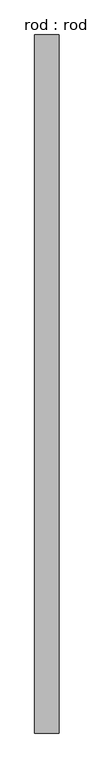
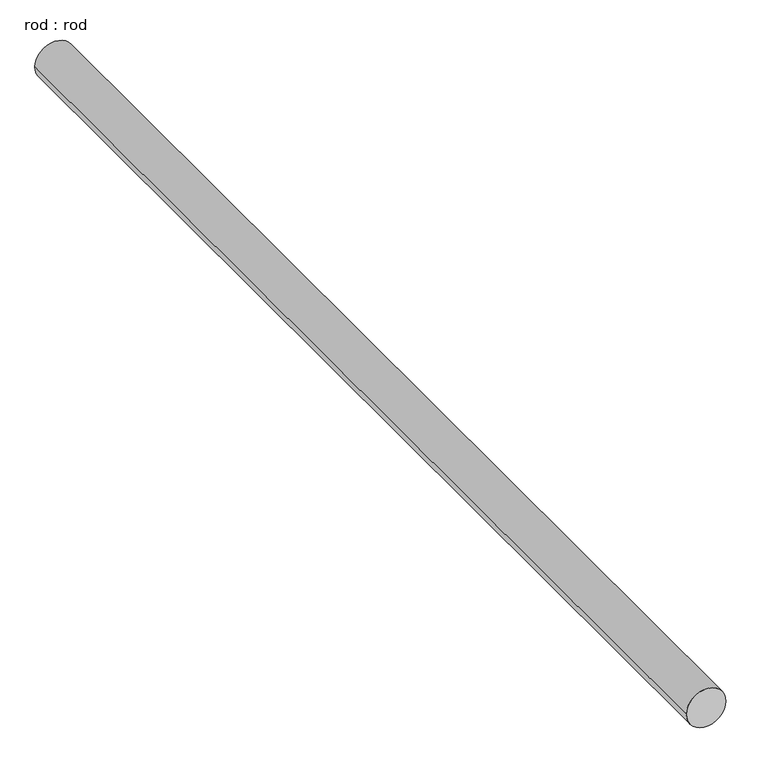
"""IFC4 building model written with IfcOpenShell, lengths in millimetres: proxy geometry, rod : rod."""

import ifcopenshell
import ifcopenshell.guid

model = None  # the IFC model being written
_history = None  # IfcOwnerHistory: only IFC2X3 demands one
_inside = {}  # id of a spatial element -> (the spatial element, [elements in it])
_under = {}  # id of a project, library or spatial element -> (it, [spatial elements below it])
_declared = {}  # id of a project -> (the project, [libraries it declares])
_typed = {}  # id of a type object -> (the type object, [elements of that type])
_made_of = {}  # id of a material, layer set ... -> (it, [elements and type objects made of it])


def new_model(schema):
    """Start an empty IFC model of exactly this schema.

    Asked for "IFC4X3", IfcOpenShell would pick the latest addendum, in which some entities
    have other attributes; the version numbers below select the first issue.
    IFC2X3 requires an IfcOwnerHistory on every rooted entity: one is made here for all.
    """
    global model, _history
    if schema == "IFC4X3":
        model = ifcopenshell.file(schema_version=(4, 3, 0, 0))
    else:
        model = ifcopenshell.file(schema=schema)
    _inside.clear()
    _under.clear()
    _declared.clear()
    _typed.clear()
    _made_of.clear()
    _history = None
    if model.schema == "IFC2X3":
        org = make("IfcOrganization", Name="unknown")
        user = make(
            "IfcPersonAndOrganization",
            ThePerson=make("IfcPerson", FamilyName="unknown"),
            TheOrganization=org,
        )
        app = make(
            "IfcApplication",
            ApplicationDeveloper=org,
            Version="unknown",
            ApplicationFullName="unknown",
            ApplicationIdentifier="unknown",
        )
        _history = make(
            "IfcOwnerHistory",
            OwningUser=user,
            OwningApplication=app,
            ChangeAction="ADDED",
            CreationDate=0,
        )
    return model


def make(cls, **values):
    """One entity of the class cls with the attributes given. An attribute that is None is left unset."""
    return model.create_entity(
        cls, **{name: value for name, value in values.items() if value is not None}
    )


def rooted(cls, **values):
    """An entity with a GlobalId (a new one), such as an element, a storey or a relation."""
    return make(cls, GlobalId=ifcopenshell.guid.new(), OwnerHistory=_history, **values)


def si_unit(unit_type, name, prefix=None):
    """IfcSIUnit, for example si_unit("LENGTHUNIT", "METRE", prefix="MILLI")."""
    return make("IfcSIUnit", UnitType=unit_type, Prefix=prefix, Name=name)


def assignment(units):
    """IfcUnitAssignment: the units of a project."""
    return None if units is None else make("IfcUnitAssignment", Units=units)


def point(xyz):
    """IfcCartesianPoint."""
    return None if xyz is None else make("IfcCartesianPoint", Coordinates=xyz)


def direction(xyz):
    """IfcDirection."""
    return None if xyz is None else make("IfcDirection", DirectionRatios=xyz)


def frame(location, z_axis=None, x_axis=None):
    """IfcAxis2Placement3D, a coordinate frame: its origin and axes. An axis left out is left unset."""
    return make(
        "IfcAxis2Placement3D",
        Location=point(location),
        Axis=direction(z_axis),
        RefDirection=direction(x_axis),
    )


def frame_2d(location, x_axis=None):
    """IfcAxis2Placement2D, a coordinate frame in the plane: its origin and x axis."""
    return make(
        "IfcAxis2Placement2D", Location=point(location), RefDirection=direction(x_axis)
    )


def origin():
    """The frame at (0, 0, 0) with its axes left unset."""
    return frame((0.0, 0.0, 0.0))


def place(relative_to, where):
    """IfcLocalPlacement: puts the frame where relative to a parent placement (None: the world)."""
    return make(
        "IfcLocalPlacement", PlacementRelTo=relative_to, RelativePlacement=where
    )


def context(
    kind, dimensions, precision=None, world=None, true_north=None, identifier=None
):
    """IfcGeometricRepresentationContext, for example the 3D "Model" context."""
    return make(
        "IfcGeometricRepresentationContext",
        ContextIdentifier=identifier,
        ContextType=kind,
        CoordinateSpaceDimension=dimensions,
        Precision=precision,
        WorldCoordinateSystem=world,
        TrueNorth=true_north,
    )


def project(units=None, contexts=None):
    """IfcProject with its units and contexts."""
    return rooted(
        "IfcProject",
        Name="project",
        RepresentationContexts=contexts,
        UnitsInContext=assignment(units),
    )


def spatial(cls, under=None, at=None, **own):
    """A site, building, storey or space (cls), placed at a placement, below another one or the project."""
    s = rooted(cls, ObjectPlacement=at, **own)
    if under is not None:
        _under.setdefault(under.id(), (under, []))[1].append(s)
    return s


def circle_curve(where, radius):
    """IfcCircle in the frame where."""
    return make("IfcCircle", Position=where, Radius=radius)


def trimmed(basis, trim1, trim2, sense, master):
    """IfcTrimmedCurve: the piece of a basis curve between two trims."""
    return make(
        "IfcTrimmedCurve",
        BasisCurve=basis,
        Trim1=trim1,
        Trim2=trim2,
        SenseAgreement=sense,
        MasterRepresentation=master,
    )


def segment(curve, same_sense, transition):
    """IfcCompositeCurveSegment."""
    return make(
        "IfcCompositeCurveSegment",
        Transition=transition,
        SameSense=same_sense,
        ParentCurve=curve,
    )


def composite_curve(segments, self_intersect=None):
    """IfcCompositeCurve: segments joined end to end."""
    return make("IfcCompositeCurve", Segments=segments, SelfIntersect=self_intersect)


def outline(outer, holes=None, kind="AREA"):
    """IfcArbitraryClosedProfileDef: a profile drawn as a closed curve; with holes, ...WithVoids."""
    if holes is None:
        return make("IfcArbitraryClosedProfileDef", ProfileType=kind, OuterCurve=outer)
    return make(
        "IfcArbitraryProfileDefWithVoids",
        ProfileType=kind,
        OuterCurve=outer,
        InnerCurves=holes,
    )


def extrude(swept, where, along, depth):
    """IfcExtrudedAreaSolid: the profile swept, set in the frame where, extruded along a direction by depth."""
    return make(
        "IfcExtrudedAreaSolid",
        SweptArea=swept,
        Position=where,
        ExtrudedDirection=direction(along),
        Depth=depth,
    )


def shape(context_of_items, identifier, shape_type, items):
    """IfcShapeRepresentation: the items that make up one representation, for example the "Body"."""
    return make(
        "IfcShapeRepresentation",
        ContextOfItems=context_of_items,
        RepresentationIdentifier=identifier,
        RepresentationType=shape_type,
        Items=items,
    )


def source(mapping_origin, context_of_items, identifier, shape_type, items):
    """IfcRepresentationMap: a shape defined once, which mapped items show again and again."""
    return make(
        "IfcRepresentationMap",
        MappingOrigin=mapping_origin,
        MappedRepresentation=shape(context_of_items, identifier, shape_type, items),
    )


def transform(
    local_origin,
    x_axis=None,
    y_axis=None,
    z_axis=None,
    scale=None,
    scale2=None,
    scale3=None,
    uniform=True,
):
    """IfcCartesianTransformationOperator3D, or its non-uniform kind. x_axis, y_axis, z_axis: its Axis1, 2, 3."""
    if uniform:
        return make(
            "IfcCartesianTransformationOperator3D",
            Axis1=direction(x_axis),
            Axis2=direction(y_axis),
            LocalOrigin=point(local_origin),
            Scale=scale,
            Axis3=direction(z_axis),
        )
    return make(
        "IfcCartesianTransformationOperator3DnonUniform",
        Axis1=direction(x_axis),
        Axis2=direction(y_axis),
        LocalOrigin=point(local_origin),
        Scale=scale,
        Axis3=direction(z_axis),
        Scale2=scale2,
        Scale3=scale3,
    )


def mapped(mapping_source, mapping_target):
    """IfcMappedItem: shows the shape of a source again, moved by a transform."""
    return make(
        "IfcMappedItem", MappingSource=mapping_source, MappingTarget=mapping_target
    )


def made_of(thing, what):
    """Note that an element or type object is made of a material, layer set ...; save() writes the relation."""
    if what is not None:
        _made_of.setdefault(what.id(), (what, []))[1].append(thing)
    return thing


def element(
    cls,
    number,
    at=None,
    inside=None,
    cuts=None,
    type_object=None,
    material=None,
    context=None,
    identifier="Body",
    shape_type=None,
    held_by="IfcProductDefinitionShape",
    body=None,
    shapes=None,
    **own,
):
    """One element of the class cls, such as IfcWall. Its Tag is "e" and its number.

    at: its placement. inside: the storey or other place that contains it. cuts: it is an
    opening in that element (IfcRelVoidsElement). A single representation is given by context,
    identifier, shape_type and body (its items); several are given by shapes. held_by: the class
    of the entity that holds the representations. save() writes the other relations.
    """
    e = rooted(cls, Tag="e%d" % number, ObjectPlacement=at, **own)
    if body is not None:
        shapes = [shape(context, identifier, shape_type, body)]
    if shapes is not None:
        e.Representation = make(held_by, Representations=shapes)
    if inside is not None:
        _inside.setdefault(inside.id(), (inside, []))[1].append(e)
    if cuts is not None:
        rooted(
            "IfcRelVoidsElement", RelatingBuildingElement=cuts, RelatedOpeningElement=e
        )
    if type_object is not None:
        _typed.setdefault(type_object.id(), (type_object, []))[1].append(e)
    return made_of(e, material)


def aggregate(whole, parts):
    """IfcRelAggregates: a whole, such as a stair, and the parts it consists of."""
    return rooted("IfcRelAggregates", RelatingObject=whole, RelatedObjects=parts)


def save(model, path):
    """Write the relations noted so far, then the file.

    IfcRelAggregates (storeys below a building ...), IfcRelContainedInSpatialStructure (elements
    in a storey), IfcRelDefinesByType, IfcRelAssociatesMaterial and IfcRelDeclares: one each for
    every whole, place, type object, material and project.
    """
    for whole, parts in _under.values():
        aggregate(whole, parts)
    for where, things in _inside.values():
        rooted(
            "IfcRelContainedInSpatialStructure",
            RelatedElements=things,
            RelatingStructure=where,
        )
    for kind, things in _typed.values():
        rooted("IfcRelDefinesByType", RelatedObjects=things, RelatingType=kind)
    for what, things in _made_of.values():
        rooted("IfcRelAssociatesMaterial", RelatedObjects=things, RelatingMaterial=what)
    for by, libraries in _declared.values():
        rooted("IfcRelDeclares", RelatingContext=by, RelatedDefinitions=libraries)
    model.write(path)


def rod_rod_01fecffa(model_context):
    return source(origin(), model_context, "Body", "SweptSolid", [
        extrude(outline(composite_curve([segment(trimmed(circle_curve(frame_2d((0.0108462, 0.0)), 200.0), [point((0.0108462, 200.0))], [point((0.0108462, -200.0))], False, "CARTESIAN"), True, "CONTINUOUS"), segment(trimmed(circle_curve(frame_2d((0.0108462, 0.0)), 200.0), [point((0.0108462, -200.0))], [point((0.0108462, 200.0))], False, "CARTESIAN"), True, "CONTINUOUS")], self_intersect=False)), frame((0.0, -1594.7713847, 0.0), z_axis=(0.0, 1.0, 0.0), x_axis=(0.0, 0.0, 1.0)), (0.0, 0.0, 1.0), 11375.0),
    ])


if __name__ == "__main__":
    model = new_model("IFC4")
    model_context = context("Model", 3, world=origin())
    ifc_project = project(units=[si_unit("LENGTHUNIT", "METRE", prefix="MILLI")], contexts=[model_context])
    site = spatial("IfcSite", under=ifc_project)
    building = spatial("IfcBuilding", under=site)
    placement = place(None, origin())
    rod_rod_shape = rod_rod_01fecffa(model_context)
    element("IfcBuildingElementProxy", 1, Name="rod : rod", ObjectType="rod : rod", at=placement, inside=building, context=model_context, shape_type="MappedRepresentation", body=[
        mapped(rod_rod_shape, transform((0.0, 0.0, 0.0), x_axis=(1.0, 0.0, 0.0), y_axis=(0.0, 1.0, 0.0), z_axis=(0.0, 0.0, 1.0))),
    ])
    save(model, "model.ifc")

# Revit data of these elements
# Type "rod : rod"
#   Default Elevation = 0
